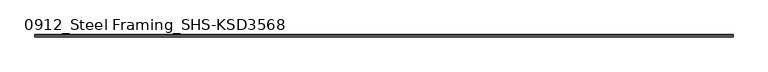
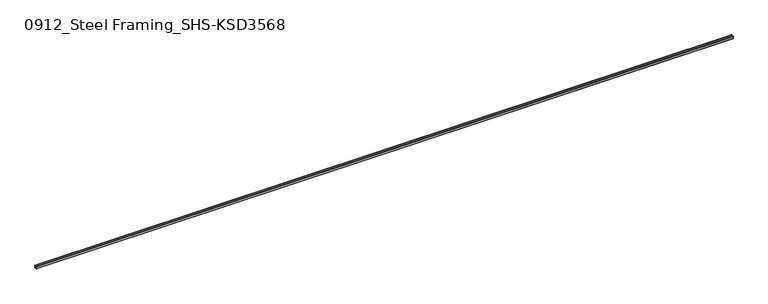
"""IFC4 building model written with IfcOpenShell, lengths in millimetres: beam geometry, 0912_Steel Framing_SHS-KSD3568 : H_SB_ASB_SHS-150x150x6."""

from ifc_helpers import new_model, si_unit, point, frame, frame_2d, origin, place, context, project, spatial, polyline, circle_curve, trimmed, segment, composite_curve, outline, extrude, source, transform, mapped, element, save


def beam_0912_steel_framing_shs_ksd3568_4780d030(model_context):
    return source(origin(), model_context, "Body", "SweptSolid", [
        extrude(outline(composite_curve([segment(polyline([(75.0, 63.0), (75.0, -63.0)]), True, "CONTINUOUS"), segment(trimmed(circle_curve(frame_2d((63.0, -63.0)), 12.0), [point((75.0, -63.0))], [point((63.0, -75.0))], False, "CARTESIAN"), True, "CONTINUOUS"), segment(polyline([(63.0, -75.0), (-63.0, -75.0)]), True, "CONTINUOUS"), segment(trimmed(circle_curve(frame_2d((-63.0, -63.0)), 12.0), [point((-63.0, -75.0))], [point((-75.0, -63.0))], False, "CARTESIAN"), True, "CONTINUOUS"), segment(polyline([(-75.0, -63.0), (-75.0, 63.0)]), True, "CONTINUOUS"), segment(trimmed(circle_curve(frame_2d((-63.0, 63.0)), 12.0), [point((-75.0, 63.0))], [point((-63.0, 75.0))], False, "CARTESIAN"), True, "CONTINUOUS"), segment(polyline([(-63.0, 75.0), (63.0, 75.0)]), True, "CONTINUOUS"), segment(trimmed(circle_curve(frame_2d((63.0, 63.0)), 12.0), [point((63.0, 75.0))], [point((75.0, 63.0))], False, "CARTESIAN"), True, "CONTINUOUS")], self_intersect=False), holes=[composite_curve([segment(trimmed(circle_curve(frame_2d((-63.0, 63.0)), 6.0), [point((-63.0, 69.0))], [point((-69.0, 63.0))], True, "CARTESIAN"), True, "CONTINUOUS"), segment(polyline([(-69.0, 63.0), (-69.0, -63.0)]), True, "CONTINUOUS"), segment(trimmed(circle_curve(frame_2d((-63.0, -63.0)), 6.0), [point((-69.0, -63.0))], [point((-63.0, -69.0))], True, "CARTESIAN"), True, "CONTINUOUS"), segment(polyline([(-63.0, -69.0), (63.0, -69.0)]), True, "CONTINUOUS"), segment(trimmed(circle_curve(frame_2d((63.0, -63.0)), 6.0), [point((63.0, -69.0))], [point((69.0, -63.0))], True, "CARTESIAN"), True, "CONTINUOUS"), segment(polyline([(69.0, -63.0), (69.0, 63.0)]), True, "CONTINUOUS"), segment(trimmed(circle_curve(frame_2d((63.0, 63.0)), 6.0), [point((69.0, 63.0))], [point((63.0, 69.0))], True, "CARTESIAN"), True, "CONTINUOUS"), segment(polyline([(63.0, 69.0), (-63.0, 69.0)]), True, "CONTINUOUS")], self_intersect=False)]), frame((-20622.5, 0.0, 0.0), z_axis=(1.0, 0.0, 0.0), x_axis=(0.0, 1.0, 0.0)), (0.0, 0.0, 1.0), 41245.0),
    ])


if __name__ == "__main__":
    model = new_model("IFC4")
    model_context = context("Model", 3, world=origin())
    ifc_project = project(units=[si_unit("LENGTHUNIT", "METRE", prefix="MILLI")], contexts=[model_context])
    site = spatial("IfcSite", under=ifc_project)
    building = spatial("IfcBuilding", under=site)
    placement = place(None, origin())
    beam_0912_steel_framing_shs_ksd3568_shape = beam_0912_steel_framing_shs_ksd3568_4780d030(model_context)
    element("IfcBeam", 1, ObjectType="0912_Steel Framing_SHS-KSD3568 : H_SB_ASB_SHS-150x150x6", at=placement, inside=building, context=model_context, shape_type="MappedRepresentation", body=[
        mapped(beam_0912_steel_framing_shs_ksd3568_shape, transform((0.0, 0.0, 0.0), x_axis=(1.0, 0.0, 0.0), y_axis=(0.0, 1.0, 0.0), z_axis=(0.0, 0.0, 1.0))),
    ])
    save(model, "model.ifc")

# Revit data of these elements
# Type "0912_Steel Framing_SHS-KSD3568 : H_SB_ASB_SHS-150x150x6"
#   H_WM Code_1 = "S01AA002-00001 | Main Steel Structure Fabrication Work | Shelter/Building | Medium Steel - Standard (90KG/M>Weight≥30KG/M) | Material: (   )"
#   H_WM Code_2 = "S03AA028-00001 | Main Steel Structure Erection Work | Shelter/Building | Medium Steel (90KG/M>Weight≥30KG/M) | Material: (   )"
#   H_WM Code_3 = "S01AA010-00001 | Main Steel Structure Fabrication Work | Shelter/Building | Steel Painting/Coating | for Non-Fireproofed Steel Surface, Surface Preparation, Primer, Second & Final Coat | Material: (   )"
#   H_Q'ty Cal Type Tag = "SB-Q2"
#   Perimeter = 0.60 m²/m
#   Nominal Weight = 26.40 kgf/m
#   Length [instance default] = 1.0000 m
#   b = 0.1500 m
#   h = 0.1500 m
#   tr = 0.0120 m
#   t = 0.0060 m
#   A = 28.36 m²
#   Structural Material [instance default] = Steel, 45-345
# Element 1 (IfcBeam, "0912_Steel Framing_SHS-KSD3568 : H_SB_ASB_SHS-150x150x6")
#   Structural Material = none
# Materials
#   "Steel, 45-345": class "Metal", colour RGB 189 187 185, transparency 0, Description = "Steel 345 MPa", Cost = 0
